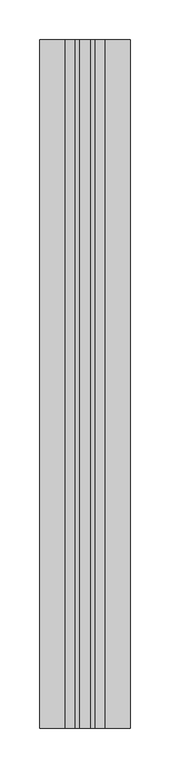
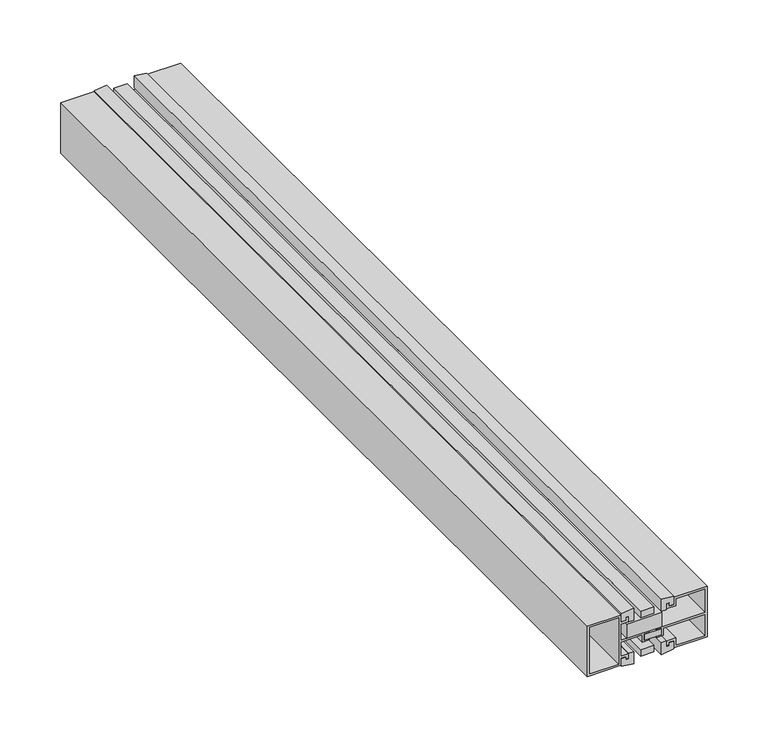
"""IFC4 building model written with IfcOpenShell, lengths in millimetres: proxy geometry, Generic Models 3:Generic Models 1:3:Generic Models 1:3 : Generic Models 3:Generic Models 1:300625:336034:Generic Models 1:3:Generic Models 1:3 : Generic Models 3:Generic Models 1:300625:336034 : Generic Models 3:Generic Models 1:3:Generic Models 1:3 : Generic Models 3:Generic Models 1:300625:336034:2 : Generic Models 3:Generic Models 1:3:Generic Models 1:3 : Generic Models 3:Generic Models 1:300625:336034:Generic Models 1:3:Generic Models 1:3 : Generic Models 3:Generic Models 1:300625:336034 : Generic Models 3:Generic Models 1:3:Generic Models 1:3 : Generic Models 3:Generic Models 1:300625:336034:301191."""

from ifc_helpers import new_model, si_unit, frame, origin, place, context, project, spatial, polyline, outline, extrude, source, transform, mapped, element, save


def generic_models_aaff98bf(model_context):
    return source(origin(), model_context, "Body", "SweptSolid", [
        extrude(outline(polyline([(560311.6698356, -573515.9126607), (560298.9698356, -573515.9126607), (560298.9698356, -572647.5501607), (560311.6698356, -572647.5501607), (560311.6698356, -573515.9126607)])), frame((0.0, 0.0, 2441.2521298), z_axis=(0.0, 0.0, 1.0), x_axis=(1.0, 0.0, 0.0)), (0.0, 0.0, 1.0), 6.3435484),
        extrude(outline(polyline([(2437.3831629, 560280.3335989), (2435.9222961, 560292.2314048), (2447.9925532, 560292.2314048), (2447.9925532, 560287.4773489), (2442.2790126, 560287.4773489), (2442.2790126, 560284.6316707), (2445.2228723, 560284.6316707), (2445.2228723, 560280.3335989), (2437.3831629, 560280.3335989)])), frame((0.0, -573515.9126607, 0.0), z_axis=(0.0, 1.0, 0.0), x_axis=(0.0, 0.0, 1.0)), (0.0, 0.0, 1.0), 868.3625),
        extrude(outline(polyline([(2442.2790126, 560323.1623223), (2447.9925532, 560323.1623223), (2447.9925532, 560318.4082665), (2435.9222961, 560318.4082665), (2437.3831629, 560330.3060723), (2445.2228723, 560330.3060723), (2445.2228723, 560326.0080005), (2442.2790126, 560326.0080005), (2442.2790126, 560323.1623223)])), frame((0.0, -573515.9126607, 0.0), z_axis=(0.0, 1.0, 0.0), x_axis=(0.0, 0.0, 1.0)), (0.0, 0.0, 1.0), 868.3625),
        extrude(outline(polyline([(560319.1513516, -573515.9126607), (560285.8645165, -573515.9126607), (560285.8645165, -572647.5501607), (560319.1513516, -572647.5501607), (560319.1513516, -573515.9126607)])), frame((0.0, 0.0, 2463.7831117), z_axis=(0.0, 0.0, 1.0), x_axis=(1.0, 0.0, 0.0)), (0.0, 0.0, 1.0), 14.2115027),
        extrude(outline(polyline([(560318.4673755, -573515.9126607), (560302.3559394, -573515.9126607), (560302.3559394, -572647.5501607), (560318.4673755, -572647.5501607), (560318.4673755, -573515.9126607)])), frame((0.0, 0.0, 2455.803391), z_axis=(0.0, 0.0, 1.0), x_axis=(1.0, 0.0, 0.0)), (0.0, 0.0, 1.0), 6.0797872),
        extrude(outline(polyline([(560311.6698356, -573515.9126607), (560298.9698356, -573515.9126607), (560298.9698356, -572647.5501607), (560311.6698356, -572647.5501607), (560311.6698356, -573515.9126607)])), frame((0.0, 0.0, 2479.9705452), z_axis=(0.0, 0.0, 1.0), x_axis=(1.0, 0.0, 0.0)), (0.0, 0.0, 1.0), 6.3435484),
        extrude(outline(polyline([(2485.2872108, 560287.4773489), (2479.5736702, 560287.4773489), (2479.5736702, 560292.2314048), (2491.6439273, 560292.2314048), (2490.1830605, 560280.3335989), (2482.3433511, 560280.3335989), (2482.3433511, 560284.6316707), (2485.2872108, 560284.6316707), (2485.2872108, 560287.4773489)])), frame((0.0, -573515.9126607, 0.0), z_axis=(0.0, 1.0, 0.0), x_axis=(0.0, 0.0, 1.0)), (0.0, 0.0, 1.0), 868.3625),
        extrude(outline(polyline([(2490.1830605, 560330.3060723), (2491.6439273, 560318.4082665), (2479.5736702, 560318.4082665), (2479.5736702, 560323.1623223), (2485.2872108, 560323.1623223), (2485.2872108, 560326.0080005), (2482.3433511, 560326.0080005), (2482.3433511, 560330.3060723), (2490.1830605, 560330.3060723)])), frame((0.0, -573515.9126607, 0.0), z_axis=(0.0, 1.0, 0.0), x_axis=(0.0, 0.0, 1.0)), (0.0, 0.0, 1.0), 868.3625),
        extrude(outline(polyline([(2438.4, 560248.1867239), (2438.4, 560279.9367239), (2445.6197473, 560279.9367239), (2445.6197473, 560285.0285457), (2443.1005159, 560285.0285457), (2443.1005159, 560287.0804739), (2447.6716755, 560287.0804739), (2447.6716755, 560279.9367239), (2461.8831782, 560279.9367239), (2461.8831782, 560300.4560059), (2454.5114362, 560300.4560059), (2454.5114362, 560307.2197691), (2455.803391, 560307.2197691), (2455.803391, 560302.3559394), (2461.8831782, 560302.3559394), (2461.8831782, 560307.2197691), (2463.7831117, 560307.2197691), (2463.7831117, 560279.9367239), (2479.9705452, 560279.9367239), (2479.9705452, 560287.0804739), (2484.8903358, 560287.0804739), (2484.8903358, 560285.0285457), (2481.9464761, 560285.0285457), (2481.9464761, 560279.9367239), (2489.1662234, 560279.9367239), (2489.1662234, 560248.1867239), (2438.4, 560248.1867239)]), holes=[polyline([(2487.2662899, 560278.0367904), (2440.2999335, 560278.0367904), (2440.2999335, 560250.6946362), (2487.2662899, 560250.6946362), (2487.2662899, 560278.0367904)])]), frame((0.0, -573515.9126607, 0.0), z_axis=(0.0, 1.0, 0.0), x_axis=(0.0, 0.0, 1.0)), (0.0, 0.0, 1.0), 868.3625),
        extrude(outline(polyline([(2484.8903358, 560325.6111255), (2484.8903358, 560323.5591973), (2479.9705452, 560323.5591973), (2479.9705452, 560332.6028808), (2487.2564243, 560332.6028808), (2487.2564243, 560360.5107931), (2463.7831117, 560360.5107931), (2463.7831117, 560313.6035457), (2461.8831782, 560313.6035457), (2461.8831782, 560318.4673755), (2455.803391, 560318.4673755), (2455.803391, 560313.6035457), (2454.5114362, 560313.6035457), (2454.5114362, 560320.367309), (2461.8831782, 560320.367309), (2461.8831782, 560360.5107931), (2440.3222126, 560360.5107931), (2440.3222126, 560332.6028808), (2447.6716755, 560332.6028808), (2447.6716755, 560323.5591973), (2443.1005159, 560323.5591973), (2443.1005159, 560325.6111255), (2445.6197473, 560325.6111255), (2445.6197473, 560330.7029473), (2438.4, 560330.7029473), (2438.4, 560362.4867239), (2489.1662234, 560362.4867239), (2489.1662234, 560330.7029473), (2481.9464761, 560330.7029473), (2481.9464761, 560325.6111255), (2484.8903358, 560325.6111255)])), frame((0.0, -573515.9126607, 0.0), z_axis=(0.0, 1.0, 0.0), x_axis=(0.0, 0.0, 1.0)), (0.0, 0.0, 1.0), 868.3625),
    ])


if __name__ == "__main__":
    model = new_model("IFC4")
    model_context = context("Model", 3, world=origin())
    ifc_project = project(units=[si_unit("LENGTHUNIT", "METRE", prefix="MILLI")], contexts=[model_context])
    site = spatial("IfcSite", under=ifc_project)
    building = spatial("IfcBuilding", under=site)
    placement = place(None, origin())
    generic_models_shape = generic_models_aaff98bf(model_context)
    element("IfcBuildingElementProxy", 1, Name="Generic Models 3:Generic Models 1:3:Generic Models 1:3 : Generic Models 3:Generic Models 1:300625:336034:Generic Models 1:3:Generic Models 1:3 : Generic Models 3:Generic Models 1:300625:336034 : Generic Models 3:Generic Models 1:3:Generic Models 1:3 : Generic Models 3:Generic Models 1:300625:336034:2 : Generic Models 3:Generic Models 1:3:Generic Models 1:3 : Generic Models 3:Generic Models 1:300625:336034:Generic Models 1:3:Generic Models 1:3 : Generic Models 3:Generic Models 1:300625:336034 : Generic Models 3:Generic Models 1:3:Generic Models 1:3 : Generic Models 3:Generic Models 1:300625:336034:301191", ObjectType="Generic Models 3:Generic Models 1:3:Generic Models 1:3 : Generic Models 3:Generic Models 1:300625:336034:Generic Models 1:3:Generic Models 1:3 : Generic Models 3:Generic Models 1:300625:336034 : Generic Models 3:Generic Models 1:3:Generic Models 1:3 : Generic Models 3:Generic Models 1:300625:336034:2 : Generic Models 3:Generic Models 1:3:Generic Models 1:3 : Generic Models 3:Generic Models 1:300625:336034:Generic Models 1:3:Generic Models 1:3 : Generic Models 3:Generic Models 1:300625:336034 : Generic Models 3:Generic Models 1:3:Generic Models 1:3 : Generic Models 3:Generic Models 1:300625:336034:301191", at=placement, inside=building, context=model_context, shape_type="MappedRepresentation", body=[
        mapped(generic_models_shape, transform((0.0, 0.0, 0.0), x_axis=(1.0, 0.0, 0.0), y_axis=(0.0, 1.0, 0.0), z_axis=(0.0, 0.0, 1.0))),
    ])
    save(model, "model.ifc")

# Revit data of these elements
# Type "Generic Models 3:Generic Models 1:3:Generic Models 1:3 : Generic Models 3:Generic Models 1:300625:336034:Generic Models 1:3:Generic Models 1:3 : Generic Models 3:Generic Models 1:300625:336034 : Generic Models 3:Generic Models 1:3:Generic Models 1:3 : Generic Models 3:Generic Models 1:300625:336034:2 : Generic Models 3:Generic Models 1:3:Generic Models 1:3 : Generic Models 3:Generic Models 1:300625:336034:Generic Models 1:3:Generic Models 1:3 : Generic Models 3:Generic Models 1:300625:336034 : Generic Models 3:Generic Models 1:3:Generic Models 1:3 : Generic Models 3:Generic Models 1:300625:336034:301191"
#   NameOverride = "Generic Models 3:Generic Models 1:3:Generic Models 1:3 : Generic Models 3:Generic Models 1:300625:336034:Generic Models 1:3:Generic Models 1:3 : Generic Models 3:Generic Models 1:300625:336034 : Generic Models 3:Generic Models 1:3:Generic Models 1:3 : Generic Models 3:Generic Models 1:300625:336034:301191"
#   ObjectTypeOverride = "Generic Models 1:3:Generic Models 1:3 : Generic Models 3:Generic Models 1:300625:336034 : Generic Models 3:Generic Models 1:3:Generic Models 1:3 : Generic Models 3:Generic Models 1:300625:336034"
#   Reference = "Generic Models 1"
#   Tag = "301191"
# Element 1 (IfcBuildingElementProxy, "Generic Models 3:Generic Models 1:3:Generic Models 1:3 : Generic Models 3:Generic Models 1:300625:336034:Generic Models 1:3:Generic Models 1:3 : Generic Models 3:Generic Models 1:300625:336034 : Generic Models 3:Generic Models 1:3:Generic Models 1:3 : Generic Models 3:Generic Models 1:300625:336034:2 : Generic Models 3:Generic Models 1:3:Generic Models 1:3 : Generic Models 3:Generic Models 1:300625:336034:Generic Models 1:3:Generic Models 1:3 : Generic Models 3:Generic Models 1:300625:336034 : Generic Models 3:Generic Models 1:3:Generic Models 1:3 : Generic Models 3:Generic Models 1:300625:336034:301191")
#   Materials on its faces: "THERMAL BROKEN ALUMINUM STOREFRONT"
# Materials
#   "THERMAL BROKEN ALUMINUM STOREFRONT": class "Unassigned", colour RGB 244 244 244, transparency 0, Cost = 0
